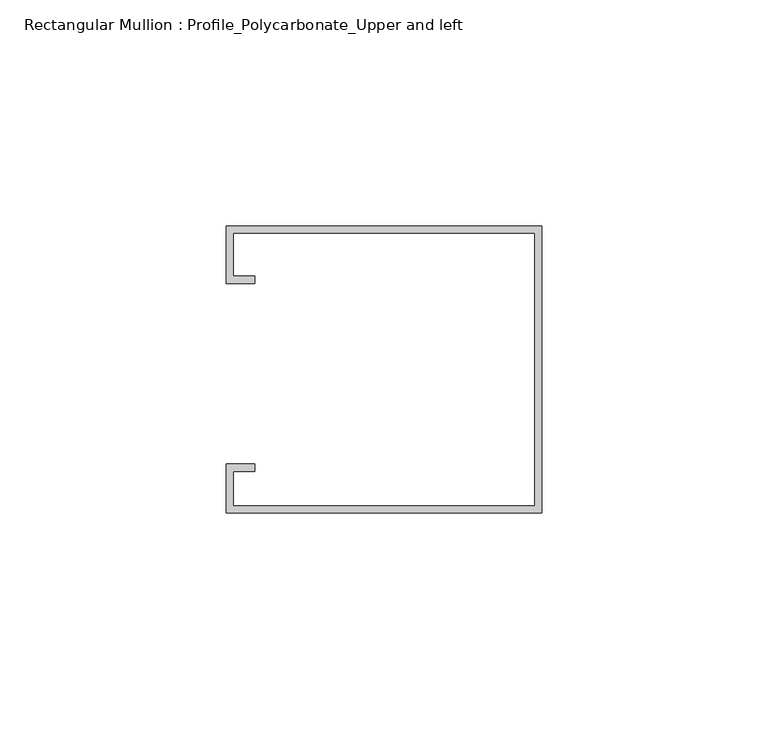
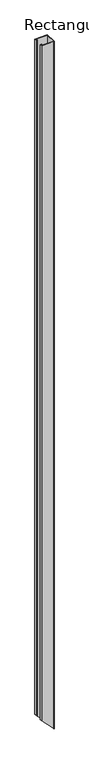
"""IFC4 building model written with IfcOpenShell, lengths in millimetres: member geometry, Rectangular Mullion : Profile_Polycarbonate_Upper and left."""

from ifc_helpers import new_model, si_unit, origin, place, context, project, spatial, faceted_brep, source, transform, mapped, element, save


def rectangular_mullion_profile_polycarbonate_upper_and_left_522ce224(model_context):
    return source(origin(), model_context, "Body", "Brep", [
        faceted_brep([(0.0, 32.7, 0.0), (-69.85, 32.7, 0.0), (-69.85, 20.0, 0.0), (-63.5, 20.0, 0.0), (-63.5, 21.5875, 0.0), (-68.2625, 21.5875, 0.0), (-68.2625, 31.1125, 0.0), (-1.5875, 31.1125, 0.0), (-1.5875, -29.2125, 0.0), (-68.2625, -29.2125, 0.0), (-68.2625, -21.5875, 0.0), (-63.5, -21.5875, 0.0), (-63.5, -20.0, 0.0), (-69.85, -20.0, 0.0), (-69.85, -30.8, 0.0), (0.0, -30.8, 0.0), (0.0, 32.7, -4041.1959545), (-69.85, 32.7, -3968.3749305), (-69.85, 20.0, -3968.3749305), (-63.5, 20.0, -3974.9950236), (-63.5, 21.5875, -3974.9950236), (-68.2625, 21.5875, -3970.0299537), (-68.2625, 31.1125, -3970.0299537), (-1.5875, 31.1125, -4039.5409312), (-1.5875, -29.2125, -4039.5409312), (-68.2625, -29.2125, -3970.0299537), (-68.2625, -21.5875, -3970.0299537), (-63.5, -21.5875, -3974.9950236), (-63.5, -20.0, -3974.9950236), (-69.85, -20.0, -3968.3749305), (-69.85, -30.8, -3968.3749305), (0.0, -30.8, -4041.1959545)], [[[0, 1, 2, 3, 4, 5, 6, 7, 8, 9, 10, 11, 12, 13, 14, 15]], [[1, 0, 16, 17]], [[2, 1, 17, 18]], [[3, 2, 18, 19]], [[4, 3, 19, 20]], [[5, 4, 20, 21]], [[6, 5, 21, 22]], [[7, 6, 22, 23]], [[8, 7, 23, 24]], [[9, 8, 24, 25]], [[10, 9, 25, 26]], [[11, 10, 26, 27]], [[12, 11, 27, 28]], [[13, 12, 28, 29]], [[14, 13, 29, 30]], [[15, 14, 30, 31]], [[0, 15, 31, 16]], [[16, 31, 30, 29, 28, 27, 26, 25, 24, 23, 22, 21, 20, 19, 18, 17]]]),
    ])


if __name__ == "__main__":
    model = new_model("IFC4")
    model_context = context("Model", 3, world=origin())
    ifc_project = project(units=[si_unit("LENGTHUNIT", "METRE", prefix="MILLI")], contexts=[model_context])
    site = spatial("IfcSite", under=ifc_project)
    building = spatial("IfcBuilding", under=site)
    placement = place(None, origin())
    rectangular_mullion_profile_polycarbonate_upper_and_left_shape = rectangular_mullion_profile_polycarbonate_upper_and_left_522ce224(model_context)
    element("IfcMember", 1, ObjectType="Rectangular Mullion : Profile_Polycarbonate_Upper and left", at=placement, inside=building, context=model_context, shape_type="MappedRepresentation", body=[
        mapped(rectangular_mullion_profile_polycarbonate_upper_and_left_shape, transform((0.0, 0.0, 0.0), x_axis=(1.0, 0.0, 0.0), y_axis=(0.0, 1.0, 0.0), z_axis=(0.0, 0.0, 1.0))),
    ])
    save(model, "model.ifc")

# Revit data of these elements
# Type "Rectangular Mullion : Profile_Polycarbonate_Upper and left"
#   built-in parameter 1007322 = 0.208333 (stored number, unit not read)
#   built-in parameter 1007321 = 0.00520833 (stored number, unit not read)
#   built-in parameter 1007320 = 0 (stored number, unit not read)
